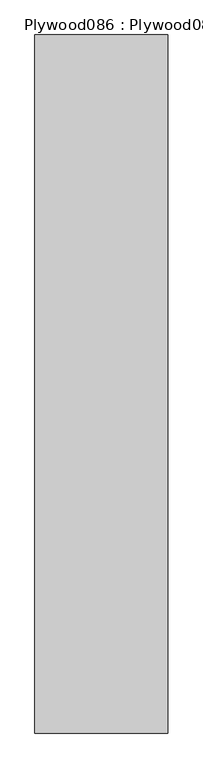
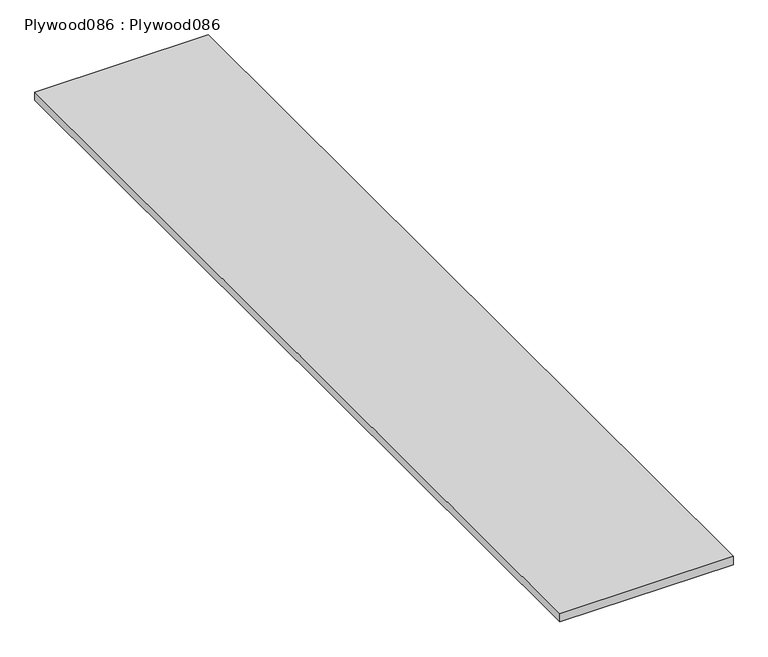
"""IFC4 building model written with IfcOpenShell, lengths in millimetres: proxy geometry, Plywood086 : Plywood086."""

from ifc_helpers import new_model, si_unit, frame, origin, place, context, project, spatial, polyline, outline, extrude, source, transform, mapped, element, save


def plywood086_plywood086_98180dae(model_context):
    return source(origin(), model_context, "Body", "SweptSolid", [
        extrude(outline(polyline([(-9404.3978931, 7982.1531721), (-9785.3978717, 7982.1531721), (-9785.3978717, 9982.1531721), (-9404.3978931, 9982.1531721), (-9404.3978931, 7982.1531721)])), frame((0.0, 0.0, 40080.9636365), z_axis=(0.0, 0.0, 1.0), x_axis=(1.0, 0.0, 0.0)), (0.0, 0.0, 1.0), 19.0499989),
    ])


if __name__ == "__main__":
    model = new_model("IFC4")
    model_context = context("Model", 3, world=origin())
    ifc_project = project(units=[si_unit("LENGTHUNIT", "METRE", prefix="MILLI")], contexts=[model_context])
    site = spatial("IfcSite", under=ifc_project)
    building = spatial("IfcBuilding", under=site)
    placement = place(None, origin())
    plywood086_plywood086_shape = plywood086_plywood086_98180dae(model_context)
    element("IfcBuildingElementProxy", 1, Name="Plywood086 : Plywood086", ObjectType="Plywood086 : Plywood086", at=placement, inside=building, context=model_context, shape_type="MappedRepresentation", body=[
        mapped(plywood086_plywood086_shape, transform((0.0, 0.0, 0.0), x_axis=(1.0, 0.0, 0.0), y_axis=(0.0, 1.0, 0.0), z_axis=(0.0, 0.0, 1.0))),
    ])
    save(model, "model.ifc")

# Revit data of these elements
# Type "Plywood086 : Plywood086"
#   NameOverride = "Plywood086"
# Element 1 (IfcBuildingElementProxy, "Plywood086 : Plywood086")
#   Materials on its faces: "CDX PLYWOOD -  SEE STRUCTURAL DWGS"
# Materials
#   "CDX PLYWOOD -  SEE STRUCTURAL DWGS": class "Unassigned", colour RGB 177 130 114, transparency 0, Cost = 0
